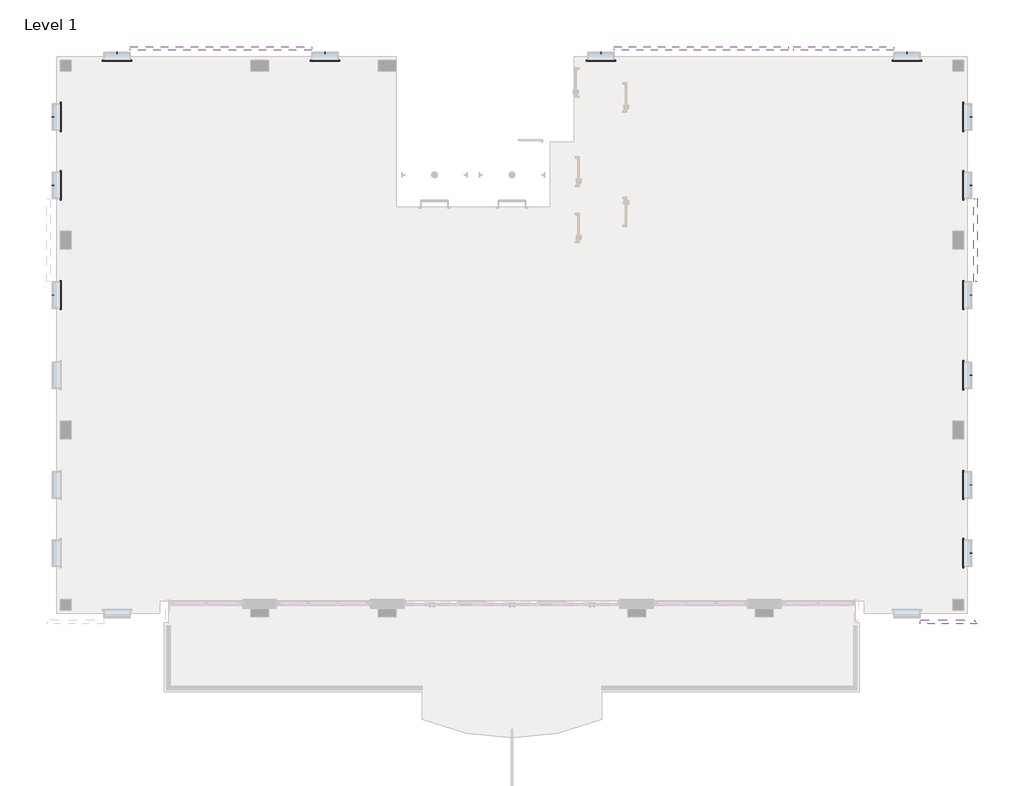
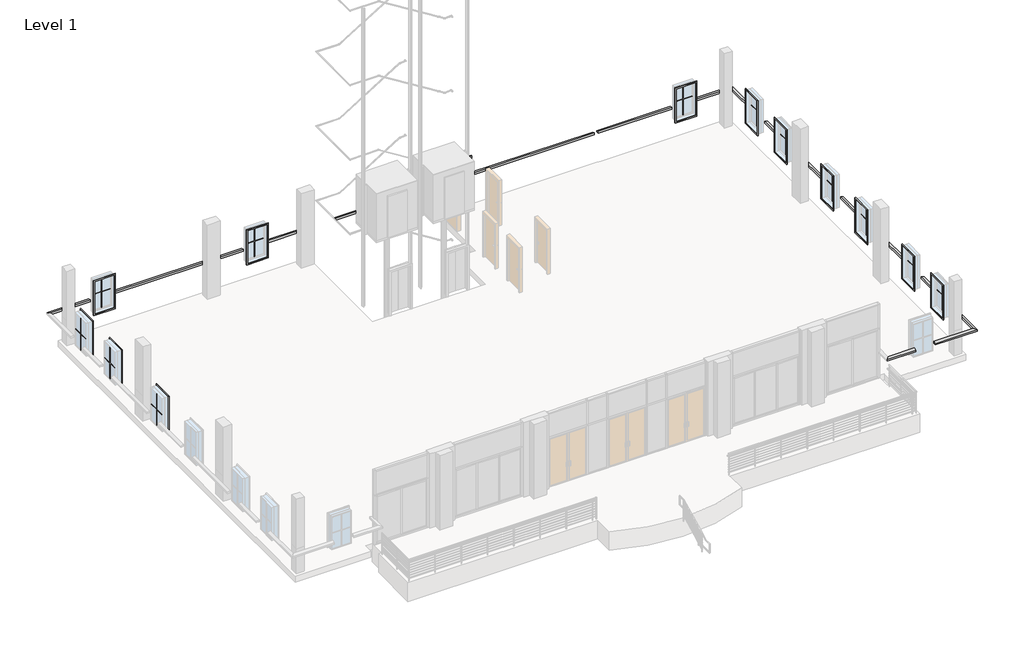
# One storey, part 5 of 5: 31 proxies.
"""IFC4 building model written with IfcOpenShell, lengths in millimetres."""

import ifcopenshell
import ifcopenshell.guid

model = None  # the IFC model being written
_history = None  # IfcOwnerHistory: only IFC2X3 demands one
_inside = {}  # id of a spatial element -> (the spatial element, [elements in it])
_under = {}  # id of a project, library or spatial element -> (it, [spatial elements below it])
_declared = {}  # id of a project -> (the project, [libraries it declares])
_typed = {}  # id of a type object -> (the type object, [elements of that type])
_made_of = {}  # id of a material, layer set ... -> (it, [elements and type objects made of it])


def new_model(schema):
    """Start an empty IFC model of exactly this schema.

    Asked for "IFC4X3", IfcOpenShell would pick the latest addendum, in which some entities
    have other attributes; the version numbers below select the first issue.
    IFC2X3 requires an IfcOwnerHistory on every rooted entity: one is made here for all.
    """
    global model, _history
    if schema == "IFC4X3":
        model = ifcopenshell.file(schema_version=(4, 3, 0, 0))
    else:
        model = ifcopenshell.file(schema=schema)
    _inside.clear()
    _under.clear()
    _declared.clear()
    _typed.clear()
    _made_of.clear()
    _history = None
    if model.schema == "IFC2X3":
        org = make("IfcOrganization", Name="unknown")
        user = make(
            "IfcPersonAndOrganization",
            ThePerson=make("IfcPerson", FamilyName="unknown"),
            TheOrganization=org,
        )
        app = make(
            "IfcApplication",
            ApplicationDeveloper=org,
            Version="unknown",
            ApplicationFullName="unknown",
            ApplicationIdentifier="unknown",
        )
        _history = make(
            "IfcOwnerHistory",
            OwningUser=user,
            OwningApplication=app,
            ChangeAction="ADDED",
            CreationDate=0,
        )
    return model


def make(cls, **values):
    """One entity of the class cls with the attributes given. An attribute that is None is left unset."""
    return model.create_entity(
        cls, **{name: value for name, value in values.items() if value is not None}
    )


def rooted(cls, **values):
    """An entity with a GlobalId (a new one), such as an element, a storey or a relation."""
    return make(cls, GlobalId=ifcopenshell.guid.new(), OwnerHistory=_history, **values)


def si_unit(unit_type, name, prefix=None):
    """IfcSIUnit, for example si_unit("LENGTHUNIT", "METRE", prefix="MILLI")."""
    return make("IfcSIUnit", UnitType=unit_type, Prefix=prefix, Name=name)


def assignment(units):
    """IfcUnitAssignment: the units of a project."""
    return None if units is None else make("IfcUnitAssignment", Units=units)


def point(xyz):
    """IfcCartesianPoint."""
    return None if xyz is None else make("IfcCartesianPoint", Coordinates=xyz)


def direction(xyz):
    """IfcDirection."""
    return None if xyz is None else make("IfcDirection", DirectionRatios=xyz)


def frame(location, z_axis=None, x_axis=None):
    """IfcAxis2Placement3D, a coordinate frame: its origin and axes. An axis left out is left unset."""
    return make(
        "IfcAxis2Placement3D",
        Location=point(location),
        Axis=direction(z_axis),
        RefDirection=direction(x_axis),
    )


def origin():
    """The frame at (0, 0, 0) with its axes left unset."""
    return frame((0.0, 0.0, 0.0))


def origin_with_axes():
    """The frame at (0, 0, 0) with the z axis (0, 0, 1) and the x axis (1, 0, 0) written out."""
    return frame((0.0, 0.0, 0.0), z_axis=(0.0, 0.0, 1.0), x_axis=(1.0, 0.0, 0.0))


def place(relative_to, where):
    """IfcLocalPlacement: puts the frame where relative to a parent placement (None: the world)."""
    return make(
        "IfcLocalPlacement", PlacementRelTo=relative_to, RelativePlacement=where
    )


def context(
    kind, dimensions, precision=None, world=None, true_north=None, identifier=None
):
    """IfcGeometricRepresentationContext, for example the 3D "Model" context."""
    return make(
        "IfcGeometricRepresentationContext",
        ContextIdentifier=identifier,
        ContextType=kind,
        CoordinateSpaceDimension=dimensions,
        Precision=precision,
        WorldCoordinateSystem=world,
        TrueNorth=true_north,
    )


def project(units=None, contexts=None):
    """IfcProject with its units and contexts."""
    return rooted(
        "IfcProject",
        Name="project",
        RepresentationContexts=contexts,
        UnitsInContext=assignment(units),
    )


def spatial(cls, under=None, at=None, **own):
    """A site, building, storey or space (cls), placed at a placement, below another one or the project."""
    s = rooted(cls, ObjectPlacement=at, **own)
    if under is not None:
        _under.setdefault(under.id(), (under, []))[1].append(s)
    return s


def polyline(points):
    """IfcPolyline through the points."""
    return make("IfcPolyline", Points=[point(p) for p in points])


def outline(outer, holes=None, kind="AREA"):
    """IfcArbitraryClosedProfileDef: a profile drawn as a closed curve; with holes, ...WithVoids."""
    if holes is None:
        return make("IfcArbitraryClosedProfileDef", ProfileType=kind, OuterCurve=outer)
    return make(
        "IfcArbitraryProfileDefWithVoids",
        ProfileType=kind,
        OuterCurve=outer,
        InnerCurves=holes,
    )


def extrude(swept, where, along, depth):
    """IfcExtrudedAreaSolid: the profile swept, set in the frame where, extruded along a direction by depth."""
    return make(
        "IfcExtrudedAreaSolid",
        SweptArea=swept,
        Position=where,
        ExtrudedDirection=direction(along),
        Depth=depth,
    )


def faces_of(points, faces, orient=None, outer=None):
    """IfcFace entities. A face is a list of loops; a loop is a list of indices into points, from 0.

    orient and outer hold one flag for each loop. By default every Orientation is true, the
    first loop of a face is its IfcFaceOuterBound and the others are IfcFaceBound.
    """
    made = []
    for i, loops in enumerate(faces):
        bounds = []
        for j, loop in enumerate(loops):
            is_outer = j == 0 if outer is None else outer[i][j]
            bounds.append(
                make(
                    "IfcFaceOuterBound" if is_outer else "IfcFaceBound",
                    Bound=make("IfcPolyLoop", Polygon=[points[k] for k in loop]),
                    Orientation=True if orient is None else orient[i][j],
                )
            )
        made.append(make("IfcFace", Bounds=bounds))
    return made


def faceted_brep(points, faces, orient=None, outer=None, voids=None):
    """IfcFacetedBrep: a solid bounded by flat faces; with voids (closed shells), ...WithVoids."""
    shared = [point(p) for p in points]
    hull = make("IfcClosedShell", CfsFaces=faces_of(shared, faces, orient, outer))
    if voids is None:
        return make("IfcFacetedBrep", Outer=hull)
    return make(
        "IfcFacetedBrepWithVoids",
        Outer=hull,
        Voids=[
            make(cls, CfsFaces=faces_of(shared, fs, o, b)) for cls, fs, o, b in voids
        ],
    )


def shape(context_of_items, identifier, shape_type, items):
    """IfcShapeRepresentation: the items that make up one representation, for example the "Body"."""
    return make(
        "IfcShapeRepresentation",
        ContextOfItems=context_of_items,
        RepresentationIdentifier=identifier,
        RepresentationType=shape_type,
        Items=items,
    )


def source(mapping_origin, context_of_items, identifier, shape_type, items):
    """IfcRepresentationMap: a shape defined once, which mapped items show again and again."""
    return make(
        "IfcRepresentationMap",
        MappingOrigin=mapping_origin,
        MappedRepresentation=shape(context_of_items, identifier, shape_type, items),
    )


def transform(
    local_origin,
    x_axis=None,
    y_axis=None,
    z_axis=None,
    scale=None,
    scale2=None,
    scale3=None,
    uniform=True,
):
    """IfcCartesianTransformationOperator3D, or its non-uniform kind. x_axis, y_axis, z_axis: its Axis1, 2, 3."""
    if uniform:
        return make(
            "IfcCartesianTransformationOperator3D",
            Axis1=direction(x_axis),
            Axis2=direction(y_axis),
            LocalOrigin=point(local_origin),
            Scale=scale,
            Axis3=direction(z_axis),
        )
    return make(
        "IfcCartesianTransformationOperator3DnonUniform",
        Axis1=direction(x_axis),
        Axis2=direction(y_axis),
        LocalOrigin=point(local_origin),
        Scale=scale,
        Axis3=direction(z_axis),
        Scale2=scale2,
        Scale3=scale3,
    )


def mapped(mapping_source, mapping_target):
    """IfcMappedItem: shows the shape of a source again, moved by a transform."""
    return make(
        "IfcMappedItem", MappingSource=mapping_source, MappingTarget=mapping_target
    )


def made_of(thing, what):
    """Note that an element or type object is made of a material, layer set ...; save() writes the relation."""
    if what is not None:
        _made_of.setdefault(what.id(), (what, []))[1].append(thing)
    return thing


def element(
    cls,
    number,
    at=None,
    inside=None,
    cuts=None,
    type_object=None,
    material=None,
    context=None,
    identifier="Body",
    shape_type=None,
    held_by="IfcProductDefinitionShape",
    body=None,
    shapes=None,
    **own,
):
    """One element of the class cls, such as IfcWall. Its Tag is "e" and its number.

    at: its placement. inside: the storey or other place that contains it. cuts: it is an
    opening in that element (IfcRelVoidsElement). A single representation is given by context,
    identifier, shape_type and body (its items); several are given by shapes. held_by: the class
    of the entity that holds the representations. save() writes the other relations.
    """
    e = rooted(cls, Tag="e%d" % number, ObjectPlacement=at, **own)
    if body is not None:
        shapes = [shape(context, identifier, shape_type, body)]
    if shapes is not None:
        e.Representation = make(held_by, Representations=shapes)
    if inside is not None:
        _inside.setdefault(inside.id(), (inside, []))[1].append(e)
    if cuts is not None:
        rooted(
            "IfcRelVoidsElement", RelatingBuildingElement=cuts, RelatedOpeningElement=e
        )
    if type_object is not None:
        _typed.setdefault(type_object.id(), (type_object, []))[1].append(e)
    return made_of(e, material)


def aggregate(whole, parts):
    """IfcRelAggregates: a whole, such as a stair, and the parts it consists of."""
    return rooted("IfcRelAggregates", RelatingObject=whole, RelatedObjects=parts)


def save(model, path):
    """Write the relations noted so far, then the file.

    IfcRelAggregates (storeys below a building ...), IfcRelContainedInSpatialStructure (elements
    in a storey), IfcRelDefinesByType, IfcRelAssociatesMaterial and IfcRelDeclares: one each for
    every whole, place, type object, material and project.
    """
    for whole, parts in _under.values():
        aggregate(whole, parts)
    for where, things in _inside.values():
        rooted(
            "IfcRelContainedInSpatialStructure",
            RelatedElements=things,
            RelatingStructure=where,
        )
    for kind, things in _typed.values():
        rooted("IfcRelDefinesByType", RelatedObjects=things, RelatingType=kind)
    for what, things in _made_of.values():
        rooted("IfcRelAssociatesMaterial", RelatedObjects=things, RelatingMaterial=what)
    for by, libraries in _declared.values():
        rooted("IfcRelDeclares", RelatingContext=by, RelatedDefinitions=libraries)
    model.write(path)


def muntin_pattern_2x2_muntin_pattern_2x2_e27c8d0d(model_context):
    return source(origin(), model_context, "Body", "SweptSolid", [
        extrude(outline(polyline([(781.05, -6.35), (781.05, -419.1), (768.35, -419.1), (768.35, -6.35), (0.0, -6.35), (0.0, 6.35), (768.35, 6.35), (768.35, 419.1), (781.05, 419.1), (781.05, 6.35), (1549.4, 6.35), (1549.4, -6.35), (781.05, -6.35)])), frame((0.0, -22.225, 0.0), z_axis=(0.0, 1.0, 0.0), x_axis=(0.0, 0.0, 1.0)), (0.0, 0.0, 1.0), 12.7),
        extrude(outline(polyline([(781.05, -6.35), (781.05, -419.1), (768.35, -419.1), (768.35, -6.35), (0.0, -6.35), (0.0, 6.35), (768.35, 6.35), (768.35, 419.1), (781.05, 419.1), (781.05, 6.35), (1549.4, 6.35), (1549.4, -6.35), (781.05, -6.35)])), frame((0.0, 9.525, 0.0), z_axis=(0.0, 1.0, 0.0), x_axis=(0.0, 0.0, 1.0)), (0.0, 0.0, 1.0), 12.7),
    ])


def muntin_pattern_2x2_muntin_pattern_2x2_e2a5a0f5(model_context):
    return source(origin(), model_context, "Body", "SweptSolid", [
        extrude(outline(polyline([(781.05, -6.35), (781.05, -419.1), (768.35, -419.1), (768.35, -6.35), (0.0, -6.35), (0.0, 6.35), (768.35, 6.35), (768.35, 419.1), (781.05, 419.1), (781.05, 6.35), (1549.4, 6.35), (1549.4, -6.35), (781.05, -6.35)])), frame((0.0, 9.525, 0.0), z_axis=(0.0, 1.0, 0.0), x_axis=(0.0, 0.0, 1.0)), (0.0, 0.0, 1.0), 12.7),
        extrude(outline(polyline([(781.05, -6.35), (781.05, -419.1), (768.35, -419.1), (768.35, -6.35), (0.0, -6.35), (0.0, 6.35), (768.35, 6.35), (768.35, 419.1), (781.05, 419.1), (781.05, 6.35), (1549.4, 6.35), (1549.4, -6.35), (781.05, -6.35)])), frame((0.0, -22.225, 0.0), z_axis=(0.0, 1.0, 0.0), x_axis=(0.0, 0.0, 1.0)), (0.0, 0.0, 1.0), 12.7),
    ])


def trim_window_interior_flat_picture_frame_9b9b1be9(model_context):
    return source(origin(), model_context, "Body", "SweptSolid", [
        extrude(outline(polyline([(501.65, 44.45), (501.65, -1670.05), (-501.65, -1670.05), (-501.65, 44.45), (501.65, 44.45)]), holes=[polyline([(444.5, -12.7), (-444.5, -12.7), (-444.5, -1612.9), (444.5, -1612.9), (444.5, -12.7)])]), origin_with_axes(), (0.0, 0.0, 1.0), 31.75),
    ])


def trim_window_interior_flat_picture_frame_cf830d55(model_context):
    return source(origin(), model_context, "Body", "SweptSolid", [
        extrude(outline(polyline([(501.65, -44.45), (-501.65, -44.45), (-501.65, 1670.05), (501.65, 1670.05), (501.65, -44.45)]), holes=[polyline([(444.5, 12.7), (444.5, 1612.9), (-444.5, 1612.9), (-444.5, 12.7), (444.5, 12.7)])]), origin_with_axes(), (0.0, 0.0, 1.0), 31.75),
    ])


model = new_model("IFC4")

# Units and contexts
model_context = context("Model", 3, world=origin())
ifc_project = project(units=[si_unit("LENGTHUNIT", "METRE", prefix="MILLI")], contexts=[model_context])

# Site, building, storey
site = spatial("IfcSite", under=ifc_project)
building = spatial("IfcBuilding", under=site)
storey = spatial("IfcBuildingStorey", under=building, Name="Level 1", Elevation=0.0)

# Proxies
placement = place(None, origin())
element("IfcBuildingElementProxy", 1, Name="Wall Sweeps", at=placement, inside=storey, context=model_context, shape_type="Brep", body=[
    faceted_brep([(-17091.6122732, 9723.3015304, 1219.2), (-16964.6122732, 9596.3015304, 1219.2), (-16964.6122732, 9596.3015304, 1320.8), (-17091.6122732, 9723.3015304, 1282.7), (-15135.8122732, 9723.3015304, 1219.2), (-15135.8122732, 9723.3015304, 1282.7), (-15135.8122732, 9596.3015304, 1320.8), (-15135.8122732, 9596.3015304, 1219.2), (-15135.8122732, 9697.9015304, 1219.2)], [[[0, 1, 2, 3]], [[4, 5, 6, 7, 8]], [[1, 0, 4, 8, 7]], [[2, 1, 7, 6]], [[3, 2, 6, 5]], [[0, 3, 5, 4]]]),
    faceted_brep([(-14221.4122732, 9723.3015304, 1219.2), (-14221.4122732, 9697.9015304, 1219.2), (-14221.4122732, 9596.3015304, 1219.2), (-14221.4122732, 9596.3015304, 1320.8), (-14221.4122732, 9723.3015304, 1282.7), (-8023.8122732, 9723.3015304, 1219.2), (-8023.8122732, 9723.3015304, 1282.7), (-8023.8122732, 9596.3015304, 1320.8), (-8023.8122732, 9596.3015304, 1219.2), (-8023.8122732, 9697.9015304, 1219.2)], [[[0, 1, 2, 3, 4]], [[5, 6, 7, 8, 9]], [[2, 1, 0, 5, 9, 8]], [[3, 2, 8, 7]], [[4, 3, 7, 6]], [[0, 4, 6, 5]]]),
    faceted_brep([(-7109.4122732, 9723.3015304, 1219.2), (-7109.4122732, 9697.9015304, 1219.2), (-7109.4122732, 9596.3015304, 1219.2), (-7109.4122732, 9596.3015304, 1320.8), (-7109.4122732, 9723.3015304, 1282.7), (-5128.2122732, 9723.3015304, 1219.2), (-5128.2122732, 9723.3015304, 1282.7), (-5128.2122732, 9596.3015304, 1320.8), (-5128.2122732, 9596.3015304, 1219.2), (-5128.2122732, 9697.9015304, 1219.2)], [[[0, 1, 2, 3, 4]], [[5, 6, 7, 8, 9]], [[2, 1, 0, 5, 9, 8]], [[3, 2, 8, 7]], [[4, 3, 7, 6]], [[0, 4, 6, 5]]]),
])
element("IfcBuildingElementProxy", 2, Name="Wall Sweeps", at=placement, inside=storey, context=model_context, shape_type="Brep", body=[
    faceted_brep([(14759.9877268, -10037.8984696, 1219.2), (14632.9877268, -9910.8984696, 1219.2), (14632.9877268, -9910.8984696, 1320.8), (14759.9877268, -10037.8984696, 1282.7), (12804.1877268, -10037.8984696, 1219.2), (12804.1877268, -10037.8984696, 1282.7), (12804.1877268, -9910.8984696, 1320.8), (12804.1877268, -9910.8984696, 1219.2), (12804.1877268, -10012.4984696, 1219.2)], [[[0, 1, 2, 3]], [[4, 5, 6, 7, 8]], [[1, 0, 4, 8, 7]], [[2, 1, 7, 6]], [[3, 2, 6, 5]], [[0, 3, 5, 4]]]),
    faceted_brep([(11889.7877268, -10037.8984696, 1219.2), (11889.7877268, -10012.4984696, 1219.2), (11889.7877268, -9910.8984696, 1219.2), (11889.7877268, -9910.8984696, 1320.8), (11889.7877268, -10037.8984696, 1282.7), (10548.0007986, -10037.8984696, 1219.2), (10548.0007986, -10037.8984696, 1282.7), (10675.0007986, -9910.8984696, 1320.8), (10675.0007986, -9910.8984696, 1219.2)], [[[0, 1, 2, 3, 4]], [[5, 6, 7, 8]], [[2, 1, 0, 5, 8]], [[3, 2, 8, 7]], [[4, 3, 7, 6]], [[0, 4, 6, 5]]]),
])
element("IfcBuildingElementProxy", 3, Name="Wall Sweeps", at=placement, inside=storey, context=model_context, shape_type="Brep", body=[
    faceted_brep([(14759.9877268, 9723.3015304, 1219.2), (14632.9877268, 9596.3015304, 1219.2), (14632.9877268, 9596.3015304, 1320.8), (14759.9877268, 9723.3015304, 1282.7), (14759.9877268, 7767.5015304, 1219.2), (14759.9877268, 7767.5015304, 1282.7), (14632.9877268, 7767.5015304, 1320.8), (14632.9877268, 7767.5015304, 1219.2), (14734.5877268, 7767.5015304, 1219.2)], [[[0, 1, 2, 3]], [[4, 5, 6, 7, 8]], [[1, 0, 4, 8, 7]], [[2, 1, 7, 6]], [[3, 2, 6, 5]], [[0, 3, 5, 4]]]),
    faceted_brep([(14759.9877268, 6853.1015304, 1219.2), (14734.5877268, 6853.1015304, 1219.2), (14632.9877268, 6853.1015304, 1219.2), (14632.9877268, 6853.1015304, 1320.8), (14759.9877268, 6853.1015304, 1282.7), (14759.9877268, 5430.7015304, 1219.2), (14759.9877268, 5430.7015304, 1282.7), (14632.9877268, 5430.7015304, 1320.8), (14632.9877268, 5430.7015304, 1219.2), (14734.5877268, 5430.7015304, 1219.2)], [[[0, 1, 2, 3, 4]], [[5, 6, 7, 8, 9]], [[2, 1, 0, 5, 9, 8]], [[3, 2, 8, 7]], [[4, 3, 7, 6]], [[0, 4, 6, 5]]]),
    faceted_brep([(14759.9877268, 4516.3015304, 1219.2), (14734.5877268, 4516.3015304, 1219.2), (14632.9877268, 4516.3015304, 1219.2), (14632.9877268, 4516.3015304, 1320.8), (14759.9877268, 4516.3015304, 1282.7), (14759.9877268, 1671.5015304, 1219.2), (14759.9877268, 1671.5015304, 1282.7), (14632.9877268, 1671.5015304, 1320.8), (14632.9877268, 1671.5015304, 1219.2), (14734.5877268, 1671.5015304, 1219.2)], [[[0, 1, 2, 3, 4]], [[5, 6, 7, 8, 9]], [[2, 1, 0, 5, 9, 8]], [[3, 2, 8, 7]], [[4, 3, 7, 6]], [[0, 4, 6, 5]]]),
    faceted_brep([(14759.9877268, 757.1015304, 1219.2), (14734.5877268, 757.1015304, 1219.2), (14632.9877268, 757.1015304, 1219.2), (14632.9877268, 757.1015304, 1320.8), (14759.9877268, 757.1015304, 1282.7), (14759.9877268, -1071.6984696, 1219.2), (14759.9877268, -1071.6984696, 1282.7), (14632.9877268, -1071.6984696, 1320.8), (14632.9877268, -1071.6984696, 1219.2), (14734.5877268, -1071.6984696, 1219.2)], [[[0, 1, 2, 3, 4]], [[5, 6, 7, 8, 9]], [[2, 1, 0, 5, 9, 8]], [[3, 2, 8, 7]], [[4, 3, 7, 6]], [[0, 4, 6, 5]]]),
    faceted_brep([(14759.9877268, -1986.0984696, 1219.2), (14734.5877268, -1986.0984696, 1219.2), (14632.9877268, -1986.0984696, 1219.2), (14632.9877268, -1986.0984696, 1320.8), (14759.9877268, -1986.0984696, 1282.7), (14759.9877268, -4830.8984696, 1219.2), (14759.9877268, -4830.8984696, 1282.7), (14632.9877268, -4830.8984696, 1320.8), (14632.9877268, -4830.8984696, 1219.2), (14734.5877268, -4830.8984696, 1219.2)], [[[0, 1, 2, 3, 4]], [[5, 6, 7, 8, 9]], [[2, 1, 0, 5, 9, 8]], [[3, 2, 8, 7]], [[4, 3, 7, 6]], [[0, 4, 6, 5]]]),
    faceted_brep([(14759.9877268, -5745.2984696, 1219.2), (14734.5877268, -5745.2984696, 1219.2), (14632.9877268, -5745.2984696, 1219.2), (14632.9877268, -5745.2984696, 1320.8), (14759.9877268, -5745.2984696, 1282.7), (14759.9877268, -7167.6984696, 1219.2), (14759.9877268, -7167.6984696, 1282.7), (14632.9877268, -7167.6984696, 1320.8), (14632.9877268, -7167.6984696, 1219.2), (14734.5877268, -7167.6984696, 1219.2)], [[[0, 1, 2, 3, 4]], [[5, 6, 7, 8, 9]], [[2, 1, 0, 5, 9, 8]], [[3, 2, 8, 7]], [[4, 3, 7, 6]], [[0, 4, 6, 5]]]),
    faceted_brep([(14759.9877268, -8082.0984696, 1219.2), (14734.5877268, -8082.0984696, 1219.2), (14632.9877268, -8082.0984696, 1219.2), (14632.9877268, -8082.0984696, 1320.8), (14759.9877268, -8082.0984696, 1282.7), (14759.9877268, -10037.8984696, 1219.2), (14759.9877268, -10037.8984696, 1282.7), (14632.9877268, -9910.8984696, 1320.8), (14632.9877268, -9910.8984696, 1219.2)], [[[0, 1, 2, 3, 4]], [[5, 6, 7, 8]], [[2, 1, 0, 5, 8]], [[3, 2, 8, 7]], [[4, 3, 7, 6]], [[0, 4, 6, 5]]]),
])
element("IfcBuildingElementProxy", 4, Name="Wall Sweeps", at=placement, inside=storey, context=model_context, shape_type="Brep", body=[
    faceted_brep([(8476.6627268, 9723.3015304, 1219.2), (8476.6627268, 9697.9015304, 1219.2), (8476.6627268, 9596.3015304, 1219.2), (8476.6627268, 9596.3015304, 1320.8), (8476.6627268, 9723.3015304, 1282.7), (11889.7877268, 9723.3015304, 1219.2), (11889.7877268, 9723.3015304, 1282.7), (11889.7877268, 9596.3015304, 1320.8), (11889.7877268, 9596.3015304, 1219.2), (11889.7877268, 9697.9015304, 1219.2)], [[[0, 1, 2, 3, 4]], [[5, 6, 7, 8, 9]], [[2, 1, 0, 5, 9, 8]], [[3, 2, 8, 7]], [[4, 3, 7, 6]], [[0, 4, 6, 5]]]),
    faceted_brep([(12804.1877268, 9723.3015304, 1219.2), (12804.1877268, 9697.9015304, 1219.2), (12804.1877268, 9596.3015304, 1219.2), (12804.1877268, 9596.3015304, 1320.8), (12804.1877268, 9723.3015304, 1282.7), (14759.9877268, 9723.3015304, 1219.2), (14759.9877268, 9723.3015304, 1282.7), (14632.9877268, 9596.3015304, 1320.8), (14632.9877268, 9596.3015304, 1219.2)], [[[0, 1, 2, 3, 4]], [[5, 6, 7, 8]], [[2, 1, 0, 5, 8]], [[3, 2, 8, 7]], [[4, 3, 7, 6]], [[0, 4, 6, 5]]]),
])
element("IfcBuildingElementProxy", 5, Name="Wall Sweeps", at=placement, inside=storey, context=model_context, shape_type="Brep", body=[
    faceted_brep([(-4934.5372732, 9723.3015304, 1219.2), (-4934.5372732, 9697.9015304, 1219.2), (-4934.5372732, 9596.3015304, 1219.2), (-4934.5372732, 9596.3015304, 1320.8), (-4934.5372732, 9723.3015304, 1282.7), (-4731.3372732, 9723.3015304, 1219.2), (-4731.3372732, 9723.3015304, 1282.7), (-4731.3372732, 9596.3015304, 1320.8), (-4731.3372732, 9596.3015304, 1219.2), (-4731.3372732, 9697.9015304, 1219.2)], [[[0, 1, 2, 3, 4]], [[5, 6, 7, 8, 9]], [[2, 1, 0, 5, 9, 8]], [[3, 2, 8, 7]], [[4, 3, 7, 6]], [[0, 4, 6, 5]]]),
    faceted_brep([(-3715.3372732, 9723.3015304, 1219.2), (-3715.3372732, 9697.9015304, 1219.2), (-3715.3372732, 9596.3015304, 1219.2), (-3715.3372732, 9596.3015304, 1320.8), (-3715.3372732, 9723.3015304, 1282.7), (1420.2252268, 9723.3015304, 1219.2), (1420.2252268, 9723.3015304, 1282.7), (1420.2252268, 9596.3015304, 1320.8), (1420.2252268, 9596.3015304, 1219.2), (1420.2252268, 9697.9015304, 1219.2)], [[[0, 1, 2, 3, 4]], [[5, 6, 7, 8, 9]], [[2, 1, 0, 5, 9, 8]], [[3, 2, 8, 7]], [[4, 3, 7, 6]], [[0, 4, 6, 5]]]),
    faceted_brep([(2334.6252268, 9723.3015304, 1219.2), (2334.6252268, 9697.9015304, 1219.2), (2334.6252268, 9596.3015304, 1219.2), (2334.6252268, 9596.3015304, 1320.8), (2334.6252268, 9723.3015304, 1282.7), (8282.9877268, 9723.3015304, 1219.2), (8282.9877268, 9723.3015304, 1282.7), (8282.9877268, 9596.3015304, 1320.8), (8282.9877268, 9596.3015304, 1219.2), (8282.9877268, 9697.9015304, 1219.2)], [[[0, 1, 2, 3, 4]], [[5, 6, 7, 8, 9]], [[2, 1, 0, 5, 9, 8]], [[3, 2, 8, 7]], [[4, 3, 7, 6]], [[0, 4, 6, 5]]]),
])
muntin_pattern_2x2_muntin_pattern_2x2_shape = muntin_pattern_2x2_muntin_pattern_2x2_e27c8d0d(model_context)
element("IfcBuildingElementProxy", 6, Name="Muntin Pattern_2x2 : Muntin Pattern_2x2", ObjectType="Muntin Pattern_2x2 : Muntin Pattern_2x2", at=placement, inside=storey, context=model_context, shape_type="MappedRepresentation", body=[
    mapped(muntin_pattern_2x2_muntin_pattern_2x2_shape, transform((12346.9877268, 9497.8765304, 850.9), x_axis=(-1.0, 0.0, 0.0), y_axis=(0.0, -1.0, 0.0), z_axis=(0.0, 0.0, 1.0))),
])
element("IfcBuildingElementProxy", 7, Name="Muntin Pattern_2x2 : Muntin Pattern_2x2", ObjectType="Muntin Pattern_2x2 : Muntin Pattern_2x2", at=placement, inside=storey, context=model_context, shape_type="MappedRepresentation", body=[
    mapped(muntin_pattern_2x2_muntin_pattern_2x2_shape, transform((1877.4252268, 9497.8765304, 850.9), x_axis=(-1.0, 0.0, 0.0), y_axis=(0.0, -1.0, 0.0), z_axis=(0.0, 0.0, 1.0))),
])
element("IfcBuildingElementProxy", 8, Name="Muntin Pattern_2x2 : Muntin Pattern_2x2", ObjectType="Muntin Pattern_2x2 : Muntin Pattern_2x2", at=placement, inside=storey, context=model_context, shape_type="MappedRepresentation", body=[
    mapped(muntin_pattern_2x2_muntin_pattern_2x2_shape, transform((-7566.6122732, 9497.8765304, 850.9), x_axis=(-1.0, 0.0, 0.0), y_axis=(0.0, -1.0, 0.0), z_axis=(0.0, 0.0, 1.0))),
])
element("IfcBuildingElementProxy", 9, Name="Muntin Pattern_2x2 : Muntin Pattern_2x2", ObjectType="Muntin Pattern_2x2 : Muntin Pattern_2x2", at=placement, inside=storey, context=model_context, shape_type="MappedRepresentation", body=[
    mapped(muntin_pattern_2x2_muntin_pattern_2x2_shape, transform((-14678.6122732, 9497.8765304, 850.9), x_axis=(-1.0, 0.0, 0.0), y_axis=(0.0, -1.0, 0.0), z_axis=(0.0, 0.0, 1.0))),
])
element("IfcBuildingElementProxy", 10, Name="Muntin Pattern_2x2 : Muntin Pattern_2x2", ObjectType="Muntin Pattern_2x2 : Muntin Pattern_2x2", at=placement, inside=storey, context=model_context, shape_type="MappedRepresentation", body=[
    mapped(muntin_pattern_2x2_muntin_pattern_2x2_shape, transform((-16866.1872732, 7310.3015304, 850.9), x_axis=(0.0, -1.0, 0.0), y_axis=(1.0, 0.0, 0.0), z_axis=(0.0, 0.0, 1.0))),
])
element("IfcBuildingElementProxy", 11, Name="Muntin Pattern_2x2 : Muntin Pattern_2x2", ObjectType="Muntin Pattern_2x2 : Muntin Pattern_2x2", at=placement, inside=storey, context=model_context, shape_type="MappedRepresentation", body=[
    mapped(muntin_pattern_2x2_muntin_pattern_2x2_shape, transform((-16866.1872732, 4973.5015304, 850.9), x_axis=(0.0, -1.0, 0.0), y_axis=(1.0, 0.0, 0.0), z_axis=(0.0, 0.0, 1.0))),
])
element("IfcBuildingElementProxy", 12, Name="Muntin Pattern_2x2 : Muntin Pattern_2x2", ObjectType="Muntin Pattern_2x2 : Muntin Pattern_2x2", at=placement, inside=storey, context=model_context, shape_type="MappedRepresentation", body=[
    mapped(muntin_pattern_2x2_muntin_pattern_2x2_shape, transform((-16866.1872732, 1214.3015304, 850.9), x_axis=(0.0, -1.0, 0.0), y_axis=(1.0, 0.0, 0.0), z_axis=(0.0, 0.0, 1.0))),
])
muntin_pattern_2x2_muntin_pattern_2x2_2_shape = muntin_pattern_2x2_muntin_pattern_2x2_e2a5a0f5(model_context)
element("IfcBuildingElementProxy", 13, Name="Muntin Pattern_2x2 : Muntin Pattern_2x2", ObjectType="Muntin Pattern_2x2 : Muntin Pattern_2x2", at=placement, inside=storey, context=model_context, shape_type="MappedRepresentation", body=[
    mapped(muntin_pattern_2x2_muntin_pattern_2x2_2_shape, transform((14534.5627268, 7310.3015304, 850.9), x_axis=(0.0, -1.0, 0.0), y_axis=(1.0, 0.0, 0.0), z_axis=(0.0, 0.0, 1.0))),
])
element("IfcBuildingElementProxy", 14, Name="Muntin Pattern_2x2 : Muntin Pattern_2x2", ObjectType="Muntin Pattern_2x2 : Muntin Pattern_2x2", at=placement, inside=storey, context=model_context, shape_type="MappedRepresentation", body=[
    mapped(muntin_pattern_2x2_muntin_pattern_2x2_2_shape, transform((14534.5627268, 4973.5015304, 850.9), x_axis=(0.0, -1.0, 0.0), y_axis=(1.0, 0.0, 0.0), z_axis=(0.0, 0.0, 1.0))),
])
element("IfcBuildingElementProxy", 15, Name="Muntin Pattern_2x2 : Muntin Pattern_2x2", ObjectType="Muntin Pattern_2x2 : Muntin Pattern_2x2", at=placement, inside=storey, context=model_context, shape_type="MappedRepresentation", body=[
    mapped(muntin_pattern_2x2_muntin_pattern_2x2_2_shape, transform((14534.5627268, 1214.3015304, 850.9), x_axis=(0.0, -1.0, 0.0), y_axis=(1.0, 0.0, 0.0), z_axis=(0.0, 0.0, 1.0))),
])
element("IfcBuildingElementProxy", 16, Name="Muntin Pattern_2x2 : Muntin Pattern_2x2", ObjectType="Muntin Pattern_2x2 : Muntin Pattern_2x2", at=placement, inside=storey, context=model_context, shape_type="MappedRepresentation", body=[
    mapped(muntin_pattern_2x2_muntin_pattern_2x2_2_shape, transform((14534.5627268, -1528.8984696, 850.9), x_axis=(0.0, -1.0, 0.0), y_axis=(1.0, 0.0, 0.0), z_axis=(0.0, 0.0, 1.0))),
])
element("IfcBuildingElementProxy", 17, Name="Muntin Pattern_2x2 : Muntin Pattern_2x2", ObjectType="Muntin Pattern_2x2 : Muntin Pattern_2x2", at=placement, inside=storey, context=model_context, shape_type="MappedRepresentation", body=[
    mapped(muntin_pattern_2x2_muntin_pattern_2x2_2_shape, transform((14534.5627268, -5288.0984696, 850.9), x_axis=(0.0, -1.0, 0.0), y_axis=(1.0, 0.0, 0.0), z_axis=(0.0, 0.0, 1.0))),
])
element("IfcBuildingElementProxy", 18, Name="Muntin Pattern_2x2 : Muntin Pattern_2x2", ObjectType="Muntin Pattern_2x2 : Muntin Pattern_2x2", at=placement, inside=storey, context=model_context, shape_type="MappedRepresentation", body=[
    mapped(muntin_pattern_2x2_muntin_pattern_2x2_2_shape, transform((14534.5627268, -7624.8984696, 850.9), x_axis=(0.0, -1.0, 0.0), y_axis=(1.0, 0.0, 0.0), z_axis=(0.0, 0.0, 1.0))),
])
trim_window_interior_flat_picture_frame_shape = trim_window_interior_flat_picture_frame_9b9b1be9(model_context)
element("IfcBuildingElementProxy", 19, Name="Trim-Window-Interior-Flat : Picture Frame", ObjectType="Trim-Window-Interior-Flat : Picture Frame", at=placement, inside=storey, context=model_context, shape_type="MappedRepresentation", body=[
    mapped(trim_window_interior_flat_picture_frame_shape, transform((12346.9877268, 9259.7515304, 2438.4), x_axis=(1.0, 0.0, 0.0), y_axis=(0.0, 0.0, 1.0), z_axis=(0.0, -1.0, 0.0))),
])
element("IfcBuildingElementProxy", 20, Name="Trim-Window-Interior-Flat : Picture Frame", ObjectType="Trim-Window-Interior-Flat : Picture Frame", at=placement, inside=storey, context=model_context, shape_type="MappedRepresentation", body=[
    mapped(trim_window_interior_flat_picture_frame_shape, transform((1877.4252268, 9259.7515304, 2438.4), x_axis=(1.0, 0.0, 0.0), y_axis=(0.0, 0.0, 1.0), z_axis=(0.0, -1.0, 0.0))),
])
element("IfcBuildingElementProxy", 21, Name="Trim-Window-Interior-Flat : Picture Frame", ObjectType="Trim-Window-Interior-Flat : Picture Frame", at=placement, inside=storey, context=model_context, shape_type="MappedRepresentation", body=[
    mapped(trim_window_interior_flat_picture_frame_shape, transform((-7566.6122732, 9259.7515304, 2438.4), x_axis=(1.0, 0.0, 0.0), y_axis=(0.0, 0.0, 1.0), z_axis=(0.0, -1.0, 0.0))),
])
element("IfcBuildingElementProxy", 22, Name="Trim-Window-Interior-Flat : Picture Frame", ObjectType="Trim-Window-Interior-Flat : Picture Frame", at=placement, inside=storey, context=model_context, shape_type="MappedRepresentation", body=[
    mapped(trim_window_interior_flat_picture_frame_shape, transform((-14678.6122732, 9259.7515304, 2438.4), x_axis=(1.0, 0.0, 0.0), y_axis=(0.0, 0.0, 1.0), z_axis=(0.0, -1.0, 0.0))),
])
element("IfcBuildingElementProxy", 23, Name="Trim-Window-Interior-Flat : Picture Frame", ObjectType="Trim-Window-Interior-Flat : Picture Frame", at=placement, inside=storey, context=model_context, shape_type="MappedRepresentation", body=[
    mapped(trim_window_interior_flat_picture_frame_shape, transform((-16628.0622732, 7310.3015304, 2438.4), x_axis=(0.0, 1.0, 0.0), y_axis=(0.0, 0.0, 1.0), z_axis=(1.0, 0.0, 0.0))),
])
element("IfcBuildingElementProxy", 24, Name="Trim-Window-Interior-Flat : Picture Frame", ObjectType="Trim-Window-Interior-Flat : Picture Frame", at=placement, inside=storey, context=model_context, shape_type="MappedRepresentation", body=[
    mapped(trim_window_interior_flat_picture_frame_shape, transform((-16628.0622732, 4973.5015304, 2438.4), x_axis=(0.0, 1.0, 0.0), y_axis=(0.0, 0.0, 1.0), z_axis=(1.0, 0.0, 0.0))),
])
element("IfcBuildingElementProxy", 25, Name="Trim-Window-Interior-Flat : Picture Frame", ObjectType="Trim-Window-Interior-Flat : Picture Frame", at=placement, inside=storey, context=model_context, shape_type="MappedRepresentation", body=[
    mapped(trim_window_interior_flat_picture_frame_shape, transform((-16628.0622732, 1214.3015304, 2438.4), x_axis=(0.0, 1.0, 0.0), y_axis=(0.0, 0.0, 1.0), z_axis=(1.0, 0.0, 0.0))),
])
trim_window_interior_flat_picture_frame_2_shape = trim_window_interior_flat_picture_frame_cf830d55(model_context)
element("IfcBuildingElementProxy", 26, Name="Trim-Window-Interior-Flat : Picture Frame", ObjectType="Trim-Window-Interior-Flat : Picture Frame", at=placement, inside=storey, context=model_context, shape_type="MappedRepresentation", body=[
    mapped(trim_window_interior_flat_picture_frame_2_shape, transform((14296.4377268, 7310.3015304, 2438.4), x_axis=(0.0, 1.0, 0.0), y_axis=(0.0, 0.0, -1.0), z_axis=(-1.0, 0.0, 0.0))),
])
element("IfcBuildingElementProxy", 27, Name="Trim-Window-Interior-Flat : Picture Frame", ObjectType="Trim-Window-Interior-Flat : Picture Frame", at=placement, inside=storey, context=model_context, shape_type="MappedRepresentation", body=[
    mapped(trim_window_interior_flat_picture_frame_2_shape, transform((14296.4377268, 4973.5015304, 2438.4), x_axis=(0.0, 1.0, 0.0), y_axis=(0.0, 0.0, -1.0), z_axis=(-1.0, 0.0, 0.0))),
])
element("IfcBuildingElementProxy", 28, Name="Trim-Window-Interior-Flat : Picture Frame", ObjectType="Trim-Window-Interior-Flat : Picture Frame", at=placement, inside=storey, context=model_context, shape_type="MappedRepresentation", body=[
    mapped(trim_window_interior_flat_picture_frame_2_shape, transform((14296.4377268, 1214.3015304, 2438.4), x_axis=(0.0, 1.0, 0.0), y_axis=(0.0, 0.0, -1.0), z_axis=(-1.0, 0.0, 0.0))),
])
element("IfcBuildingElementProxy", 29, Name="Trim-Window-Interior-Flat : Picture Frame", ObjectType="Trim-Window-Interior-Flat : Picture Frame", at=placement, inside=storey, context=model_context, shape_type="MappedRepresentation", body=[
    mapped(trim_window_interior_flat_picture_frame_2_shape, transform((14296.4377268, -1528.8984696, 2438.4), x_axis=(0.0, 1.0, 0.0), y_axis=(0.0, 0.0, -1.0), z_axis=(-1.0, 0.0, 0.0))),
])
element("IfcBuildingElementProxy", 30, Name="Trim-Window-Interior-Flat : Picture Frame", ObjectType="Trim-Window-Interior-Flat : Picture Frame", at=placement, inside=storey, context=model_context, shape_type="MappedRepresentation", body=[
    mapped(trim_window_interior_flat_picture_frame_2_shape, transform((14296.4377268, -5288.0984696, 2438.4), x_axis=(0.0, 1.0, 0.0), y_axis=(0.0, 0.0, -1.0), z_axis=(-1.0, 0.0, 0.0))),
])
element("IfcBuildingElementProxy", 31, Name="Trim-Window-Interior-Flat : Picture Frame", ObjectType="Trim-Window-Interior-Flat : Picture Frame", at=placement, inside=storey, context=model_context, shape_type="MappedRepresentation", body=[
    mapped(trim_window_interior_flat_picture_frame_2_shape, transform((14296.4377268, -7624.8984696, 2438.4), x_axis=(0.0, 1.0, 0.0), y_axis=(0.0, 0.0, -1.0), z_axis=(-1.0, 0.0, 0.0))),
])

save(model, "model.ifc")

# Revit data of these elements
# Project information
#   Organization Name = "G3B Press"
#   Organization Description = "Paul F. Aubin Cosulting Services, Inc."
#   Building Name = "Revit Essentials for Architecture"
#   Author = "Paul F. Aubin"
#   Author Website = "https://www.paulaubin.com"
#   Copyright = "Copyright © 2020 Paul F Aubin, all rights reserved"
#   Design Option = "Main Model"
#   Project Issue Date = "8/1/2020"
#   Project Status = "Design Development"
#   Client Name = "Developing the Exterior Skin"
#   Project Address = "123 State ST\nSuite 301\nChicago, IL 60606"
#   Project Name = "10 Commercial_Complete"
#   Project Number = "2020.04A"
# Grids (mm)
#   "1": line (-22547.601, -9504.498) -> (19277.595, -9504.498)
#   "2": line (-22547.601, -3408.498) -> (19277.595, -3408.498)
#   "3": line (-22547.601, 3093.902) -> (19277.595, 3093.902)
#   "4": line (-22547.601, 9189.902) -> (19277.595, 9189.902)
#   "A": line (-16558.212, 12259.726) -> (-16558.212, -14197.104)
#   "B": line (-9801.812, 12259.726) -> (-9801.812, -14197.104)
#   "C": line (-5433.012, 12259.726) -> (-5433.012, -14197.104)
#   "D": line (3101.388, 12259.726) -> (3101.388, -14197.104)
#   "E": line (7470.188, 12259.726) -> (7470.188, -14197.104)
#   "F": line (14226.588, 12259.726) -> (14226.588, -14197.104)
#   "C.3": line (-2689.812, -15151.11) -> (-2689.812, -5965.346)
#   "C.7": line (358.188, -15151.11) -> (358.188, -5965.346)
# Type "Muntin Pattern_2x2 : Muntin Pattern_2x2"
#   Width [instance default] = 4' - 0"
#   Thickness = 0' - 0 1/2"
#   Height [instance default] = 4' - 0"
#   Distance = 0' - 0 3/4"
#   Interior Material [instance default] = none
#   Exterior Material [instance default] = none
#   Default Elevation = 0
# Type "Trim-Window-Interior-Flat : Picture Frame"
#   Trim Thickness_Picture Frame = 0' - 1 1/4"
#   Trim Width = 0' - 2 1/4"
#   Trim Thickness_with Sill = 0' - 0 3/4"
#   Sill Thickness = 0' - 1 1/4"
#   Opening Width [instance default] = 2' - 0"
#   Opening Height [instance default] = 3' - 0"
#   Default Elevation = 4' - 0"
#   Sill = no
#   Picture Frame = yes
#   Trim Material [instance default] = none
# Elements 1, 2, 3, 4, 5 (IfcBuildingElementProxy)
#   Phase Created = New Construction
#   Materials on its faces: "Concrete - Cast-in-Place Concrete"
# Elements 6, 7, 8, 9, 10, 11, 12, 13, 14, 15, 16, 17, 18 (IfcBuildingElementProxy, "Muntin Pattern_2x2 : Muntin Pattern_2x2")
#   Width = 2' - 9"
#   Height = 5' - 1"
#   Interior Material = Wood - Stained
#   Exterior Material = Clad - White
#   Phase Created = New Construction
#   Materials on its faces: "Clad - White", "Wood - Stained"
# Elements 19, 20, 21, 22, 23, 24, 25, 26, 27, 28, 29, 30, 31 (IfcBuildingElementProxy, "Trim-Window-Interior-Flat : Picture Frame")
#   Opening Width = 3' - 0"
#   Opening Height = 5' - 4"
#   Trim Material = Wood - Stained
#   Phase Created = New Construction
#   Materials on its faces: "Wood - Stained"
# Materials
#   "Concrete - Cast-in-Place Concrete": class "Concrete", colour RGB 192 192 192, transparency 0, Cost = 0
#   "Clad - White": class "Wood", colour RGB 242 242 238, transparency 0, Cost = 0
#   "Wood - Stained": class "Wood", colour RGB 224 178 126, transparency 0, Cost = 0
